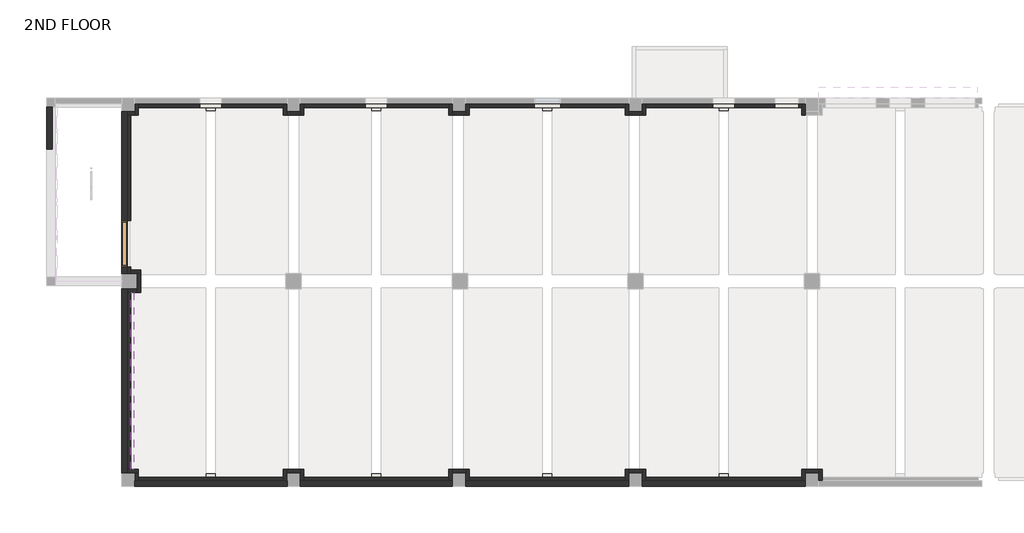
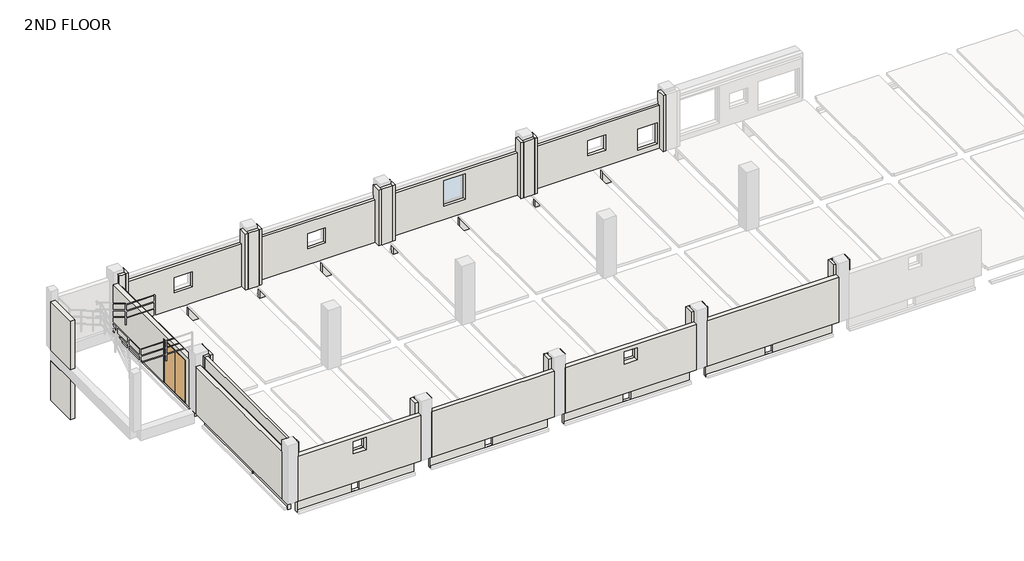
# One storey, part 1 of 7: 60 walls, 1 door.
# Revit data of these elements (continued)
# Element 1 (IfcDoor, "Double Door_Steel : H_DR_AR B12_Door_Double_W2100xH2580_No FR_SD-5")
#   Phase Created = New Construction
# Elements 2, 3, 4, 5 (IfcWall, "H_WA_AR B02_Ext Wall RC-AG_T250_W1")
#   Comments = ""
#   Top Offset = -800 mm
#   Base Offset = 0 mm
#   wall height = 2700 mm
#   Phase Created = New Construction
#   Base Constraint = 2ND FLOOR
#   Top Constraint = 3RD FLOOR
#   Materials on its faces: "Concrete_f'c=28MPa(Cylender)"
# Elements 6, 7 (IfcWall, "H_WA_AR B02_Ext Wall RC-AG_T250_W1")
#   Comments = ""
#   Top Offset = -700 mm
#   Base Offset = 0 mm
#   wall height = 2800 mm
#   Phase Created = New Construction
#   Base Constraint = 2ND FLOOR
#   Top Constraint = 3RD FLOOR
#   Materials on its faces: "Concrete_f'c=28MPa(Cylender)"
# Element 8 (IfcWall, "H_WA_AR B02_Ext Wall RC-AG_T250_W1")
#   Comments = ""
#   built-in parameter 1001111 = -3010 mm
#   Top Offset = -4150 mm
#   Base Offset = -3010 mm
#   wall height = 2360 mm
#   Phase Created = New Construction
#   Base Constraint = 2ND FLOOR
#   Top Constraint = 3RD FLOOR
#   Materials on its faces: "Concrete_f'c=28MPa(Cylender)"
# Element 9 (IfcWall, "H_WA_AR B02_Ext Wall RC-AG_T250_W1")
#   Comments = ""
#   built-in parameter 1001111 = -50 mm
#   Top Offset = -650 mm
#   Base Offset = -50 mm
#   wall height = 2900 mm
#   Phase Created = New Construction
#   Base Constraint = 2ND FLOOR
#   Top Constraint = 3RD FLOOR
#   Materials on its faces: "Concrete_f'c=28MPa(Cylender)"
# Elements 10, 36, 38, 40, 42, 44, 46, 48 (IfcWall, "H_WA_AR B02_Ext Wall DY-IN_T154")
#   Top Offset = -180 mm
#   Base Offset = 0 mm
#   wall height = 3320 mm
#   Phase Created = New Construction
#   Base Constraint = 2ND FLOOR
#   Top Constraint = 3RD FLOOR
#   Materials on its faces: "00_Finish_Gypsum Board", "00_Insulation_Glass Wool", "Default Wall"
# Elements 11, 39, 43, 47 (IfcWall, "H_WA_AR B02_Ext Wall DY-IN_T154")
#   Top Offset = -945 mm
#   Base Offset = 0 mm
#   wall height = 2555 mm
#   Phase Created = New Construction
#   Base Constraint = 2ND FLOOR
#   Top Constraint = 3RD FLOOR
#   Materials on its faces: "Default Wall", "00_Finish_Gypsum Board", "00_Insulation_Glass Wool"
# Elements 12, 17 (IfcWall, "H_WA_AR B02_Ext Wall DY-IN_T154")
#   Top Offset = -845 mm
#   Base Offset = 0 mm
#   wall height = 2655 mm
#   Phase Created = New Construction
#   Base Constraint = 2ND FLOOR
#   Top Constraint = 3RD FLOOR
#   Materials on its faces: "Default Wall", "00_Insulation_Glass Wool", "00_Finish_Gypsum Board"
# Elements 13, 16, 19, 22, 26, 30, 34 (IfcWall, "H_WA_AR B02_Ext Wall DY-IN_T154")
#   Top Offset = -180 mm
#   Base Offset = 0 mm
#   wall height = 3320 mm
#   Phase Created = New Construction
#   Base Constraint = 2ND FLOOR
#   Top Constraint = 3RD FLOOR
#   Materials on its faces: "Default Wall", "00_Insulation_Glass Wool", "00_Finish_Gypsum Board"
# Elements 14, 15, 37, 41, 45 (IfcWall, "H_WA_AR B02_Ext Wall DY-IN_T154")
#   Top Offset = -180 mm
#   Base Offset = 0 mm
#   wall height = 3320 mm
#   Phase Created = New Construction
#   Base Constraint = 2ND FLOOR
#   Top Constraint = 3RD FLOOR
#   Materials on its faces: "Default Wall", "00_Finish_Gypsum Board", "00_Insulation_Glass Wool"
# Element 18 (IfcWall, "H_WA_AR B02_Ext Wall DY-IN_T154")
#   Top Offset = -180 mm
#   Base Offset = 0 mm
#   wall height = 3320 mm
#   Phase Created = New Construction
#   Base Constraint = 2ND FLOOR
#   Top Constraint = 3RD FLOOR
#   Materials on its faces: "00_Insulation_Glass Wool", "Default Wall", "00_Finish_Gypsum Board"
# Elements 20, 24, 28, 32 (IfcWall, "H_WA_AR B02_Ext Wall DY-IN_T154")
#   Top Offset = -945 mm
#   Base Offset = 0 mm
#   wall height = 2555 mm
#   Phase Created = New Construction
#   Base Constraint = 2ND FLOOR
#   Top Constraint = 3RD FLOOR
#   Materials on its faces: "Default Wall", "00_Insulation_Glass Wool", "00_Finish_Gypsum Board"
# Elements 21, 23, 25, 27, 29, 31, 33, 35 (IfcWall, "H_WA_AR B02_Ext Wall DY-IN_T154")
#   Top Offset = -180 mm
#   Base Offset = 0 mm
#   wall height = 3320 mm
#   Phase Created = New Construction
#   Base Constraint = 2ND FLOOR
#   Top Constraint = 3RD FLOOR
#   Materials on its faces: "00_Insulation_Glass Wool", "00_Finish_Gypsum Board", "Default Wall"
# Element 49 (IfcWall, "H_WA_AR B02_Ext Wall DY-IN_T154")
#   built-in parameter 1001111 = 2655 mm
#   Top Offset = -180 mm
#   Base Offset = 2655 mm
#   wall height = 665 mm
#   Phase Created = New Construction
#   Base Constraint = 2ND FLOOR
#   Top Constraint = 3RD FLOOR
#   Materials on its faces: "Default Wall", "00_Insulation_Glass Wool", "00_Finish_Gypsum Board"
# Elements 50, 51, 57 (IfcWall, "H_WA_AR B02_Ext Wall DY-IN_T154")
#   built-in parameter 1001111 = -845 mm
#   Top Offset = -150 mm
#   Base Offset = -845 mm
#   wall height = 695 mm
#   Phase Created = New Construction
#   Base Constraint = 2ND FLOOR
#   Top Constraint = 2ND FLOOR
#   Materials on its faces: "Default Wall", "00_Finish_Gypsum Board", "00_Insulation_Glass Wool"
# Elements 52, 53, 54, 55 (IfcWall, "H_WA_AR B02_Ext Wall DY-IN_T154")
#   built-in parameter 1001111 = -945 mm
#   Top Offset = -150 mm
#   Base Offset = -945 mm
#   wall height = 795 mm
#   Phase Created = New Construction
#   Base Constraint = 2ND FLOOR
#   Top Constraint = 2ND FLOOR
#   Materials on its faces: "Default Wall", "00_Insulation_Glass Wool", "00_Finish_Gypsum Board"
# Elements 56, 58, 59, 60, 61 (IfcWall, "H_WA_AR B02_Ext Wall DY-IN_T154")
#   built-in parameter 1001111 = -945 mm
#   Top Offset = -150 mm
#   Base Offset = -945 mm
#   wall height = 795 mm
#   Phase Created = New Construction
#   Base Constraint = 2ND FLOOR
#   Top Constraint = 2ND FLOOR
#   Materials on its faces: "Default Wall", "00_Finish_Gypsum Board", "00_Insulation_Glass Wool"
# Materials
#   "Concrete_f'c=28MPa(Cylender)": class "Concrete", colour RGB 176 176 176, transparency 0, Description = "Reinf. Conc.", Cost = 0, Image = Concrete.Cast-In-Place.Flat.Polished.Grey.jpg
#   "00_Finish_Paint_Vinyl Paint": class "Finish", colour RGB 128 128 64, transparency 0, Description = "Plastic", Cost = 0
#   "00_Finish_Gypsum Board": class "Finish", colour RGB 171 170 168, transparency 0, Description = "Gypsum Board", Cost = 0, Image = Finishes.Gypsum Board.Painted.White.jpg
#   "00_Insulation_Glass Wool": class "Insulation", colour RGB 200 200 140, transparency 0, Description = "Insulation(Loose)", Cost = 0
#   "Default Wall": class "Miscellaneous", colour RGB 80 80 80, transparency 0
# Room at (21273.66, -10352.652) mm, phase "New Construction", upper level "2ND FLOOR", upper offset 3500 mm, lower offset 0 mm
#   Comments = ""
#   Occupancy = "1"
#   Number = "201"
#   Name = "CABLE ROOM"
#   H_Room H or CH = 3.5 mm
# Room at (60385.767, -12489.028) mm, phase "New Construction", upper level "2ND FLOOR", upper offset 3500 mm, lower offset 0 mm
#   Comments = ""
#   Occupancy = "1"
#   Number = "203"
#   Name = "BATTERY ROOM"
#   H_Room H or CH = 3.5 mm
# Room at (52661.948, -4436.535) mm, phase "New Construction", upper level "2ND FLOOR", upper offset 3500 mm, lower offset 0 mm
#   Comments = ""
#   Occupancy = "1"
#   Number = "202"
#   Name = "STAIRCASE"
#   H_Room H or CH = 3.5 mm
